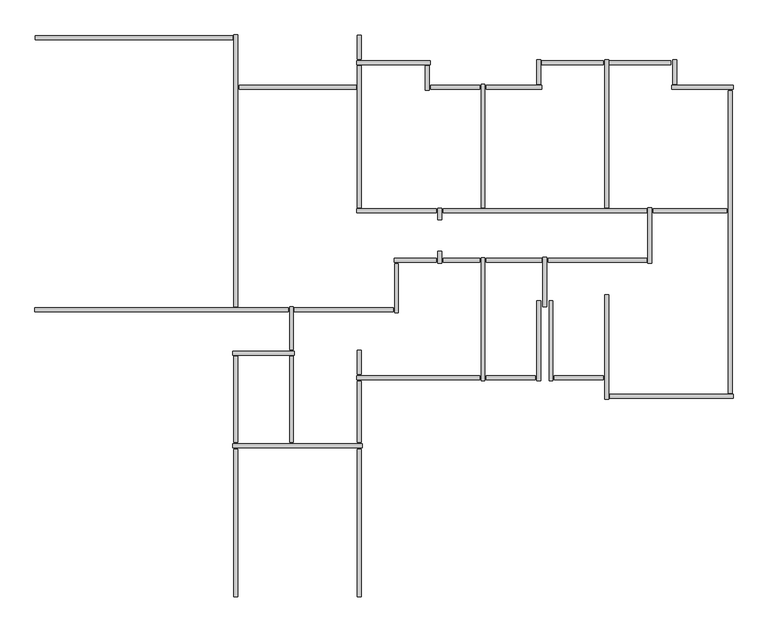
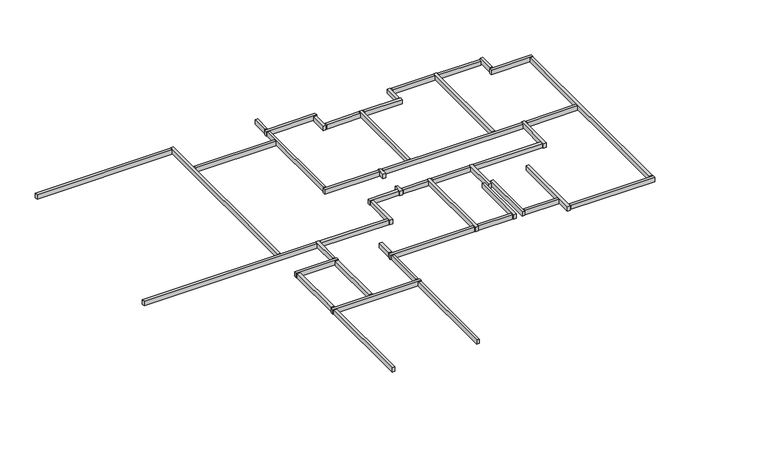
"""IFC4 building model written with IfcOpenShell, lengths in millimetres: beam geometry, Graute viga de respaldo13 : Graute viga de respaldo."""

from ifc_helpers import new_model, si_unit, frame, origin, place, context, project, spatial, polyline, outline, extrude, source, transform, mapped, element, save


def beam_b62126f0(model_context):
    return source(origin(), model_context, "Body", "SweptSolid", [
        extrude(outline(polyline([(-62804.9587292, 72814.9577736), (-62804.9587292, 72720.9577736), (-67594.9587292, 72720.9577736), (-67594.9587292, 72814.9577736), (-62804.9587292, 72814.9577736)])), frame((0.0, 0.0, 11632.9999999), z_axis=(0.0, 0.0, 1.0), x_axis=(1.0, 0.0, 0.0)), (0.0, 0.0, 1.0), 167.0),
        extrude(outline(polyline([(-59771.9587292, 62785.4278788), (-59677.9587292, 62785.4278788), (-59677.9587292, 59195.4278788), (-59771.9587292, 59195.4278788), (-59771.9587292, 62785.4278788)])), frame((0.0, 0.0, 11632.9999999), z_axis=(0.0, 0.0, 1.0), x_axis=(1.0, 0.0, 0.0)), (0.0, 0.0, 1.0), 167.0),
        extrude(outline(polyline([(-62771.9587292, 62785.4278788), (-62677.9587292, 62785.4278788), (-62677.9587292, 59195.4278788), (-62771.9587292, 59195.4278788), (-62771.9587292, 62785.4278788)])), frame((0.0, 0.0, 11632.9999999), z_axis=(0.0, 0.0, 1.0), x_axis=(1.0, 0.0, 0.0)), (0.0, 0.0, 1.0), 167.0),
        extrude(outline(polyline([(-54994.9587292, 64468.4278788), (-54994.9587292, 64562.4278788), (-53804.9587292, 64562.4278788), (-53804.9587292, 64468.4278788), (-54994.9587292, 64468.4278788)])), frame((0.0, 0.0, 11632.9999999), z_axis=(0.0, 0.0, 1.0), x_axis=(1.0, 0.0, 0.0)), (0.0, 0.0, 1.0), 167.0),
        extrude(outline(polyline([(-56644.9587292, 64468.4278788), (-56644.9587292, 64562.4278788), (-55454.9587292, 64562.4278788), (-55454.9587292, 64468.4278788), (-56644.9587292, 64468.4278788)])), frame((0.0, 0.0, 11632.9999999), z_axis=(0.0, 0.0, 1.0), x_axis=(1.0, 0.0, 0.0)), (0.0, 0.0, 1.0), 167.0),
        extrude(outline(polyline([(-52594.9587292, 68518.4278788), (-52594.9587292, 68612.4278788), (-50804.9587292, 68612.4278788), (-50804.9587292, 68518.4278788), (-52594.9587292, 68518.4278788)])), frame((0.0, 0.0, 11632.9999999), z_axis=(0.0, 0.0, 1.0), x_axis=(1.0, 0.0, 0.0)), (0.0, 0.0, 1.0), 167.0),
        extrude(outline(polyline([(-57994.9587292, 71518.4278788), (-57994.9587292, 71612.4278788), (-56804.9587292, 71612.4278788), (-56804.9587292, 71518.4278788), (-57994.9587292, 71518.4278788)])), frame((0.0, 0.0, 11632.9999999), z_axis=(0.0, 0.0, 1.0), x_axis=(1.0, 0.0, 0.0)), (0.0, 0.0, 1.0), 167.0),
        extrude(outline(polyline([(-58027.9587292, 71495.4278788), (-58121.9587292, 71495.4278788), (-58121.9587292, 72085.4278788), (-58027.9587292, 72085.4278788), (-58027.9587292, 71495.4278788)])), frame((0.0, 0.0, 11632.9999999), z_axis=(0.0, 0.0, 1.0), x_axis=(1.0, 0.0, 0.0)), (0.0, 0.0, 1.0), 167.0),
        extrude(outline(polyline([(-59794.9587292, 72118.4278788), (-59794.9587292, 72212.4278788), (-58004.9587292, 72212.4278788), (-58004.9587292, 72118.4278788), (-59794.9587292, 72118.4278788)])), frame((0.0, 0.0, 11632.9999999), z_axis=(0.0, 0.0, 1.0), x_axis=(1.0, 0.0, 0.0)), (0.0, 0.0, 1.0), 167.0),
        extrude(outline(polyline([(-57821.9587292, 68635.4278788), (-57727.9587292, 68635.4278788), (-57727.9587292, 68345.4278788), (-57821.9587292, 68345.4278788), (-57821.9587292, 68635.4278788)])), frame((0.0, 0.0, 11632.9999999), z_axis=(0.0, 0.0, 1.0), x_axis=(1.0, 0.0, 0.0)), (0.0, 0.0, 1.0), 167.0),
        extrude(outline(polyline([(-55144.9587292, 67318.4278788), (-55144.9587292, 67412.4278788), (-52754.9587292, 67412.4278788), (-52754.9587292, 67318.4278788), (-55144.9587292, 67318.4278788)])), frame((0.0, 0.0, 11632.9999999), z_axis=(0.0, 0.0, 1.0), x_axis=(1.0, 0.0, 0.0)), (0.0, 0.0, 1.0), 167.0),
        extrude(outline(polyline([(-56644.9587292, 67318.4278788), (-56644.9587292, 67412.4278788), (-55304.9587292, 67412.4278788), (-55304.9587292, 67318.4278788), (-56644.9587292, 67318.4278788)])), frame((0.0, 0.0, 11632.9999999), z_axis=(0.0, 0.0, 1.0), x_axis=(1.0, 0.0, 0.0)), (0.0, 0.0, 1.0), 167.0),
        extrude(outline(polyline([(-57694.9587292, 67318.4278788), (-57694.9587292, 67412.4278788), (-56804.9587292, 67412.4278788), (-56804.9587292, 67318.4278788), (-57694.9587292, 67318.4278788)])), frame((0.0, 0.0, 11632.9999999), z_axis=(0.0, 0.0, 1.0), x_axis=(1.0, 0.0, 0.0)), (0.0, 0.0, 1.0), 167.0),
        extrude(outline(polyline([(-57821.9587292, 67585.4278788), (-57727.9587292, 67585.4278788), (-57727.9587292, 67295.4278788), (-57821.9587292, 67295.4278788), (-57821.9587292, 67585.4278788)])), frame((0.0, 0.0, 11632.9999999), z_axis=(0.0, 0.0, 1.0), x_axis=(1.0, 0.0, 0.0)), (0.0, 0.0, 1.0), 167.0),
        extrude(outline(polyline([(-58884.9587292, 67318.4278788), (-58884.9587292, 67412.4278788), (-57854.9587292, 67412.4278788), (-57854.9587292, 67318.4278788), (-58884.9587292, 67318.4278788)])), frame((0.0, 0.0, 11632.9999999), z_axis=(0.0, 0.0, 1.0), x_axis=(1.0, 0.0, 0.0)), (0.0, 0.0, 1.0), 167.0),
        extrude(outline(polyline([(-58777.9587292, 66095.4278788), (-58871.9587292, 66095.4278788), (-58871.9587292, 67285.4278788), (-58777.9587292, 67285.4278788), (-58777.9587292, 66095.4278788)])), frame((0.0, 0.0, 11632.9999999), z_axis=(0.0, 0.0, 1.0), x_axis=(1.0, 0.0, 0.0)), (0.0, 0.0, 1.0), 167.0),
        extrude(outline(polyline([(-61304.9587292, 66118.4278788), (-61304.9587292, 66212.4278788), (-58904.9587292, 66212.4278788), (-58904.9587292, 66118.4278788), (-61304.9587292, 66118.4278788)])), frame((0.0, 0.0, 11632.9999999), z_axis=(0.0, 0.0, 1.0), x_axis=(1.0, 0.0, 0.0)), (0.0, 0.0, 1.0), 167.0),
        extrude(outline(polyline([(-56771.9587292, 67430.4278788), (-56677.9587292, 67430.4278788), (-56677.9587292, 64445.4278788), (-56771.9587292, 64445.4278788), (-56771.9587292, 67430.4278788)])), frame((0.0, 0.0, 11632.9999999), z_axis=(0.0, 0.0, 1.0), x_axis=(1.0, 0.0, 0.0)), (0.0, 0.0, 1.0), 167.0),
        extrude(outline(polyline([(-59794.9587292, 64468.4278788), (-59794.9587292, 64562.4278788), (-56804.9587292, 64562.4278788), (-56804.9587292, 64468.4278788), (-59794.9587292, 64468.4278788)])), frame((0.0, 0.0, 11632.9999999), z_axis=(0.0, 0.0, 1.0), x_axis=(1.0, 0.0, 0.0)), (0.0, 0.0, 1.0), 167.0),
        extrude(outline(polyline([(-59771.9587292, 65185.4278788), (-59677.9587292, 65185.4278788), (-59677.9587292, 64595.4278788), (-59771.9587292, 64595.4278788), (-59771.9587292, 65185.4278788)])), frame((0.0, 0.0, 11632.9999999), z_axis=(0.0, 0.0, 1.0), x_axis=(1.0, 0.0, 0.0)), (0.0, 0.0, 1.0), 167.0),
        extrude(outline(polyline([(-59677.9587292, 62945.4278788), (-59771.9587292, 62945.4278788), (-59771.9587292, 64435.4278788), (-59677.9587292, 64435.4278788), (-59677.9587292, 62945.4278788)])), frame((0.0, 0.0, 11632.9999999), z_axis=(0.0, 0.0, 1.0), x_axis=(1.0, 0.0, 0.0)), (0.0, 0.0, 1.0), 167.0),
        extrude(outline(polyline([(-62677.9587292, 62945.4278788), (-62771.9587292, 62945.4278788), (-62771.9587292, 65035.4278788), (-62677.9587292, 65035.4278788), (-62677.9587292, 62945.4278788)])), frame((0.0, 0.0, 11632.9999999), z_axis=(0.0, 0.0, 1.0), x_axis=(1.0, 0.0, 0.0)), (0.0, 0.0, 1.0), 167.0),
        extrude(outline(polyline([(-61327.9587292, 62945.4278788), (-61421.9587292, 62945.4278788), (-61421.9587292, 65035.4278788), (-61327.9587292, 65035.4278788), (-61327.9587292, 62945.4278788)])), frame((0.0, 0.0, 11632.9999999), z_axis=(0.0, 0.0, 1.0), x_axis=(1.0, 0.0, 0.0)), (0.0, 0.0, 1.0), 167.0),
        extrude(outline(polyline([(-61421.9587292, 66235.4278788), (-61327.9587292, 66235.4278788), (-61327.9587292, 65195.4278788), (-61421.9587292, 65195.4278788), (-61421.9587292, 66235.4278788)])), frame((0.0, 0.0, 11632.9999999), z_axis=(0.0, 0.0, 1.0), x_axis=(1.0, 0.0, 0.0)), (0.0, 0.0, 1.0), 167.0),
        extrude(outline(polyline([(-62644.9587292, 71518.4278788), (-62644.9587292, 71612.4278788), (-59804.9587292, 71612.4278788), (-59804.9587292, 71518.4278788), (-62644.9587292, 71518.4278788)])), frame((0.0, 0.0, 11632.9999999), z_axis=(0.0, 0.0, 1.0), x_axis=(1.0, 0.0, 0.0)), (0.0, 0.0, 1.0), 167.0),
        extrude(outline(polyline([(-59677.9587292, 68645.4278788), (-59771.9587292, 68645.4278788), (-59771.9587292, 72085.4278788), (-59677.9587292, 72085.4278788), (-59677.9587292, 68645.4278788)])), frame((0.0, 0.0, 11632.9999999), z_axis=(0.0, 0.0, 1.0), x_axis=(1.0, 0.0, 0.0)), (0.0, 0.0, 1.0), 167.0),
        extrude(outline(polyline([(-59794.9587292, 68518.4278788), (-59794.9587292, 68612.4278788), (-57854.9587292, 68612.4278788), (-57854.9587292, 68518.4278788), (-59794.9587292, 68518.4278788)])), frame((0.0, 0.0, 11632.9999999), z_axis=(0.0, 0.0, 1.0), x_axis=(1.0, 0.0, 0.0)), (0.0, 0.0, 1.0), 167.0),
        extrude(outline(polyline([(-57694.9587292, 68518.4278788), (-57694.9587292, 68612.4278788), (-52754.9587292, 68612.4278788), (-52754.9587292, 68518.4278788), (-57694.9587292, 68518.4278788)])), frame((0.0, 0.0, 11632.9999999), z_axis=(0.0, 0.0, 1.0), x_axis=(1.0, 0.0, 0.0)), (0.0, 0.0, 1.0), 167.0),
        extrude(outline(polyline([(-56771.9587292, 71635.4278788), (-56677.9587292, 71635.4278788), (-56677.9587292, 68645.4278788), (-56771.9587292, 68645.4278788), (-56771.9587292, 71635.4278788)])), frame((0.0, 0.0, 11632.9999999), z_axis=(0.0, 0.0, 1.0), x_axis=(1.0, 0.0, 0.0)), (0.0, 0.0, 1.0), 167.0),
        extrude(outline(polyline([(-55304.9587292, 71612.4278788), (-55304.9587292, 71518.4278788), (-56644.9587292, 71518.4278788), (-56644.9587292, 71612.4278788), (-55304.9587292, 71612.4278788)])), frame((0.0, 0.0, 11632.9999999), z_axis=(0.0, 0.0, 1.0), x_axis=(1.0, 0.0, 0.0)), (0.0, 0.0, 1.0), 167.0),
        extrude(outline(polyline([(-55421.9587292, 72235.4278788), (-55327.9587292, 72235.4278788), (-55327.9587292, 71645.4278788), (-55421.9587292, 71645.4278788), (-55421.9587292, 72235.4278788)])), frame((0.0, 0.0, 11632.9999999), z_axis=(0.0, 0.0, 1.0), x_axis=(1.0, 0.0, 0.0)), (0.0, 0.0, 1.0), 167.0),
        extrude(outline(polyline([(-55294.9587292, 72118.4278788), (-55294.9587292, 72212.4278788), (-53804.9587292, 72212.4278788), (-53804.9587292, 72118.4278788), (-55294.9587292, 72118.4278788)])), frame((0.0, 0.0, 11632.9999999), z_axis=(0.0, 0.0, 1.0), x_axis=(1.0, 0.0, 0.0)), (0.0, 0.0, 1.0), 167.0),
        extrude(outline(polyline([(-52165.9809043, 72212.4278788), (-52165.9809043, 72117.4278788), (-53654.9587292, 72117.4278788), (-53654.9587292, 72212.4278788), (-52165.9809043, 72212.4278788)])), frame((0.0, 0.0, 11617.1856208), z_axis=(0.0, 0.0, 1.0), x_axis=(1.0, 0.0, 0.0)), (0.0, 0.0, 1.0), 165.0),
        extrude(outline(polyline([(-50677.9587292, 64145.4278788), (-50771.9587292, 64145.4278788), (-50771.9587292, 71485.4278788), (-50677.9587292, 71485.4278788), (-50677.9587292, 64145.4278788)])), frame((0.0, 0.0, 11632.9999999), z_axis=(0.0, 0.0, 1.0), x_axis=(1.0, 0.0, 0.0)), (0.0, 0.0, 1.0), 167.0),
        extrude(outline(polyline([(-52627.9587292, 67295.4278788), (-52721.9587292, 67295.4278788), (-52721.9587292, 68640.7810915), (-52627.9587292, 68640.7810915), (-52627.9587292, 67295.4278788)])), frame((0.0, 0.0, 11632.9999999), z_axis=(0.0, 0.0, 1.0), x_axis=(1.0, 0.0, 0.0)), (0.0, 0.0, 1.0), 167.0),
        extrude(outline(polyline([(-55177.9587292, 66245.4278788), (-55271.9587292, 66245.4278788), (-55271.9587292, 67435.4278788), (-55177.9587292, 67435.4278788), (-55177.9587292, 66245.4278788)])), frame((0.0, 0.0, 11632.9999999), z_axis=(0.0, 0.0, 1.0), x_axis=(1.0, 0.0, 0.0)), (0.0, 0.0, 1.0), 167.0),
        extrude(outline(polyline([(-55027.9587292, 64445.4278788), (-55121.9587292, 64445.4278788), (-55121.9587292, 66385.4278788), (-55027.9587292, 66385.4278788), (-55027.9587292, 64445.4278788)])), frame((0.0, 0.0, 11632.9999999), z_axis=(0.0, 0.0, 1.0), x_axis=(1.0, 0.0, 0.0)), (0.0, 0.0, 1.0), 167.0),
        extrude(outline(polyline([(-55327.9587292, 64445.4278788), (-55421.9587292, 64445.4278788), (-55421.9587292, 66385.4278788), (-55327.9587292, 66385.4278788), (-55327.9587292, 64445.4278788)])), frame((0.0, 0.0, 11632.9999999), z_axis=(0.0, 0.0, 1.0), x_axis=(1.0, 0.0, 0.0)), (0.0, 0.0, 1.0), 167.0),
        extrude(outline(polyline([(-53677.9587292, 63995.4278788), (-53771.9587292, 63995.4278788), (-53771.9587292, 66535.4278788), (-53677.9587292, 66535.4278788), (-53677.9587292, 63995.4278788)])), frame((0.0, 0.0, 11632.9999999), z_axis=(0.0, 0.0, 1.0), x_axis=(1.0, 0.0, 0.0)), (0.0, 0.0, 1.0), 167.0),
        extrude(outline(polyline([(-50654.9587292, 64112.4278788), (-50654.9587292, 64018.4278788), (-53644.9587292, 64018.4278788), (-53644.9587292, 64112.4278788), (-50654.9587292, 64112.4278788)])), frame((0.0, 0.0, 11632.9999999), z_axis=(0.0, 0.0, 1.0), x_axis=(1.0, 0.0, 0.0)), (0.0, 0.0, 1.0), 167.0),
        extrude(outline(polyline([(-52121.9587292, 72235.4278788), (-52027.9587292, 72235.4278788), (-52027.9587292, 71645.4278788), (-52121.9587292, 71645.4278788), (-52121.9587292, 72235.4278788)])), frame((0.0, 0.0, 11632.9999999), z_axis=(0.0, 0.0, 1.0), x_axis=(1.0, 0.0, 0.0)), (0.0, 0.0, 1.0), 167.0),
        extrude(outline(polyline([(-52144.9587292, 71518.4278788), (-52144.9587292, 71612.4278788), (-50654.9587292, 71612.4278788), (-50654.9587292, 71518.4278788), (-52144.9587292, 71518.4278788)])), frame((0.0, 0.0, 11632.9999999), z_axis=(0.0, 0.0, 1.0), x_axis=(1.0, 0.0, 0.0)), (0.0, 0.0, 1.0), 167.0),
        extrude(outline(polyline([(-53771.9587292, 72235.4278788), (-53677.9587292, 72235.4278788), (-53677.9587292, 68645.4278788), (-53771.9587292, 68645.4278788), (-53771.9587292, 72235.4278788)])), frame((0.0, 0.0, 11632.9999999), z_axis=(0.0, 0.0, 1.0), x_axis=(1.0, 0.0, 0.0)), (0.0, 0.0, 1.0), 167.0),
        extrude(outline(polyline([(-59771.9587292, 72835.4278788), (-59677.9587292, 72835.4278788), (-59677.9587292, 72245.4278788), (-59771.9587292, 72245.4278788), (-59771.9587292, 72835.4278788)])), frame((0.0, 0.0, 11632.9999999), z_axis=(0.0, 0.0, 1.0), x_axis=(1.0, 0.0, 0.0)), (0.0, 0.0, 1.0), 167.0),
        extrude(outline(polyline([(-62794.9587292, 65068.4278788), (-62794.9587292, 65162.4278788), (-61304.9587292, 65162.4278788), (-61304.9587292, 65068.4278788), (-62794.9587292, 65068.4278788)])), frame((0.0, 0.0, 11632.9999999), z_axis=(0.0, 0.0, 1.0), x_axis=(1.0, 0.0, 0.0)), (0.0, 0.0, 1.0), 167.0),
        extrude(outline(polyline([(-62794.9587292, 62818.4278788), (-62794.9587292, 62912.4278788), (-59654.9587292, 62912.4278788), (-59654.9587292, 62818.4278788), (-62794.9587292, 62818.4278788)])), frame((0.0, 0.0, 11632.9999999), z_axis=(0.0, 0.0, 1.0), x_axis=(1.0, 0.0, 0.0)), (0.0, 0.0, 1.0), 167.0),
        extrude(outline(polyline([(-67601.7587292, 66118.4278788), (-67601.7587292, 66212.4278788), (-61454.9587292, 66212.4278788), (-61454.9587292, 66118.4278788), (-67601.7587292, 66118.4278788)])), frame((0.0, 0.0, 11632.9999999), z_axis=(0.0, 0.0, 1.0), x_axis=(1.0, 0.0, 0.0)), (0.0, 0.0, 1.0), 167.0),
        extrude(outline(polyline([(-62771.9587292, 72837.9577736), (-62677.9587292, 72837.9577736), (-62677.9587292, 66245.4278788), (-62771.9587292, 66245.4278788), (-62771.9587292, 72837.9577736)])), frame((0.0, 0.0, 11632.9999999), z_axis=(0.0, 0.0, 1.0), x_axis=(1.0, 0.0, 0.0)), (0.0, 0.0, 1.0), 167.0),
    ])


if __name__ == "__main__":
    model = new_model("IFC4")
    model_context = context("Model", 3, world=origin())
    ifc_project = project(units=[si_unit("LENGTHUNIT", "METRE", prefix="MILLI")], contexts=[model_context])
    site = spatial("IfcSite", under=ifc_project)
    building = spatial("IfcBuilding", under=site)
    placement = place(None, origin())
    beam_shape = beam_b62126f0(model_context)
    element("IfcBeam", 1, ObjectType="Graute viga de respaldo13 : Graute viga de respaldo", at=placement, inside=building, context=model_context, shape_type="MappedRepresentation", body=[
        mapped(beam_shape, transform((0.0, 0.0, 0.0), x_axis=(1.0, 0.0, 0.0), y_axis=(0.0, 1.0, 0.0), z_axis=(0.0, 0.0, 1.0))),
    ])
    save(model, "model.ifc")

# Revit data of these elements
# Element 1 (IfcBeam, "Graute viga de respaldo13 : Graute viga de respaldo")
#   Materials on its faces: "Concreto, Faixa de areia/cimento"
# Materials
#   "Concreto, Faixa de areia/cimento": class "Concreto", colour RGB 127 127 127, transparency 0, Description = "Revestimento de laje de concreto", Cost = 0
